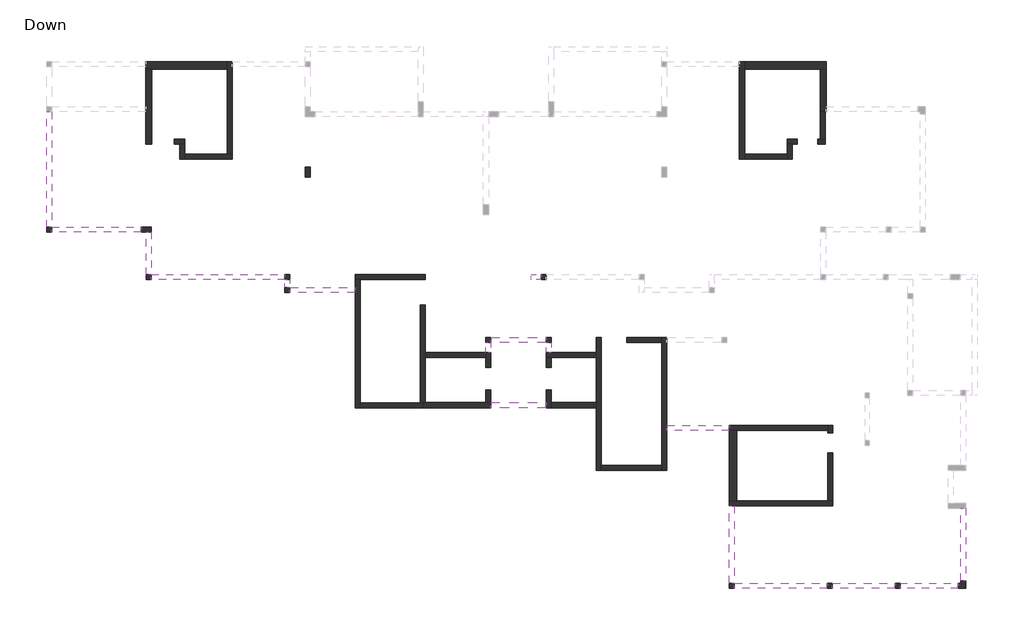
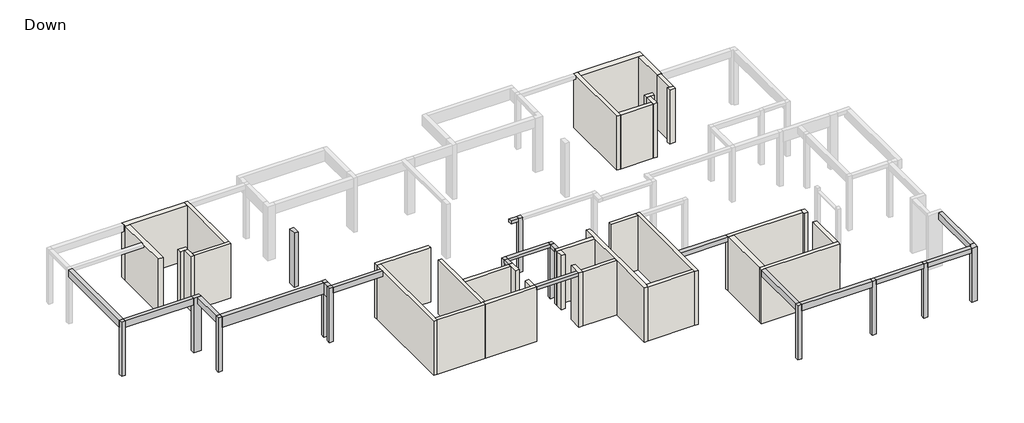
# One storey, part 1 of 2: 35 walls, 17 beams, 13 columns.
# Revit data of these elements (continued)
# Element 25 (IfcColumn, "Concrete Rectengular Column : 20/20") (continued)
#   SOFiSTiK_AMG_Adjusted = yes
#   Structural Material = Concrete
#   Phase Created = New Construction
#   Materials on its faces: "Concrete"
# Element 26 (IfcColumn, "Concrete Rectengular Column : 20/20")
#   Comments = ""
#   Mark = "C26"
#   SOFiSTiK_AMG_Comments = ""
#   SOFiSTiK_AMG_Scheduled = yes
#   SOFiSTiK_AMG_Adjusted = yes
#   Structural Material = Concrete
#   Phase Created = New Construction
#   Materials on its faces: "Concrete"
# Element 27 (IfcColumn, "Concrete Rectengular Column : 20/20")
#   Comments = ""
#   Mark = "C27"
#   SOFiSTiK_AMG_Comments = ""
#   SOFiSTiK_AMG_Scheduled = yes
#   SOFiSTiK_AMG_Adjusted = yes
#   Structural Material = Concrete
#   Phase Created = New Construction
#   Materials on its faces: "Concrete"
# Element 28 (IfcColumn, "Concrete Rectengular Column : 20/40")
#   Comments = ""
#   Mark = "C31"
#   SOFiSTiK_AMG_Comments = ""
#   SOFiSTiK_AMG_Scheduled = yes
#   SOFiSTiK_AMG_Adjusted = yes
#   Structural Material = Concrete
#   Phase Created = New Construction
#   Materials on its faces: "Concrete"
# Element 29 (IfcColumn, "Concrete Rectengular Column : 20/40")
#   Comments = ""
#   Mark = "C32"
#   SOFiSTiK_AMG_Comments = ""
#   SOFiSTiK_AMG_Scheduled = yes
#   SOFiSTiK_AMG_Adjusted = yes
#   Structural Material = Concrete
#   Phase Created = New Construction
#   Materials on its faces: "Concrete"
# Element 30 (IfcColumn, "L Column : 30/30/20/20")
#   Comments = ""
#   Mark = "C38"
#   SOFiSTiK_AMG_Comments = ""
#   SOFiSTiK_AMG_Scheduled = yes
#   SOFiSTiK_AMG_Adjusted = yes
#   Structural Material = Concrete
#   Phase Created = New Construction
# Element 31 (IfcWall, "20")
#   Comments = ""
#   Mark = "W1"
#   SOFiSTiK_AMG_Comments = ""
#   Top Offset = 0 cm
#   Base Offset = 0 cm
#   wall height = 300 cm
#   SOFiSTiK_AMG_Scheduled = yes
#   SOFiSTiK_AMG_Adjusted = yes
#   Phase Created = New Construction
#   Base Constraint = Down
#   Top Constraint = Typical Floor
#   Materials on its faces: "Concrete"
# Element 32 (IfcWall, "20")
#   Comments = ""
#   Mark = "W2"
#   SOFiSTiK_AMG_Comments = ""
#   Top Offset = 0 cm
#   Base Offset = 0 cm
#   wall height = 300 cm
#   SOFiSTiK_AMG_Scheduled = yes
#   SOFiSTiK_AMG_Adjusted = yes
#   Phase Created = New Construction
#   Base Constraint = Down
#   Top Constraint = Typical Floor
#   Materials on its faces: "Concrete"
# Element 33 (IfcWall, "20")
#   Comments = ""
#   Mark = "W3"
#   SOFiSTiK_AMG_Comments = ""
#   Top Offset = 0 cm
#   Base Offset = 0 cm
#   wall height = 300 cm
#   SOFiSTiK_AMG_Scheduled = yes
#   SOFiSTiK_AMG_Adjusted = yes
#   Phase Created = New Construction
#   Base Constraint = Down
#   Top Constraint = Typical Floor
#   Materials on its faces: "Concrete"
# Element 34 (IfcWall, "20")
#   Comments = ""
#   Mark = "W4"
#   SOFiSTiK_AMG_Comments = ""
#   Top Offset = 0 cm
#   Base Offset = 0 cm
#   wall height = 300 cm
#   SOFiSTiK_AMG_Scheduled = yes
#   SOFiSTiK_AMG_Adjusted = yes
#   Phase Created = New Construction
#   Base Constraint = Down
#   Top Constraint = Typical Floor
#   Materials on its faces: "Concrete"
# Element 35 (IfcWall, "20")
#   Comments = ""
#   Mark = "W5"
#   SOFiSTiK_AMG_Comments = ""
#   Top Offset = 0 cm
#   Base Offset = 0 cm
#   wall height = 300 cm
#   SOFiSTiK_AMG_Scheduled = yes
#   SOFiSTiK_AMG_Adjusted = yes
#   Phase Created = New Construction
#   Base Constraint = Down
#   Top Constraint = Typical Floor
#   Materials on its faces: "Concrete"
# Element 36 (IfcWall, "20")
#   Comments = ""
#   Mark = "W6"
#   SOFiSTiK_AMG_Comments = ""
#   Top Offset = 0 cm
#   Base Offset = 0 cm
#   wall height = 300 cm
#   SOFiSTiK_AMG_Scheduled = yes
#   SOFiSTiK_AMG_Adjusted = yes
#   Phase Created = New Construction
#   Base Constraint = Down
#   Top Constraint = Typical Floor
#   Materials on its faces: "Concrete"
# Element 37 (IfcWall, "20")
#   Comments = ""
#   Mark = "W7"
#   SOFiSTiK_AMG_Comments = ""
#   Top Offset = 0 cm
#   Base Offset = 0 cm
#   wall height = 300 cm
#   SOFiSTiK_AMG_Scheduled = yes
#   SOFiSTiK_AMG_Adjusted = yes
#   Phase Created = New Construction
#   Base Constraint = Down
#   Top Constraint = Typical Floor
#   Materials on its faces: "Concrete"
# Element 38 (IfcWall, "20")
#   Comments = ""
#   Mark = "W8"
#   SOFiSTiK_AMG_Comments = ""
#   Top Offset = 0 cm
#   Base Offset = 0 cm
#   wall height = 300 cm
#   SOFiSTiK_AMG_Scheduled = yes
#   SOFiSTiK_AMG_Adjusted = yes
#   Phase Created = New Construction
#   Base Constraint = Down
#   Top Constraint = Typical Floor
#   Materials on its faces: "Concrete"
# Element 39 (IfcWall, "20")
#   Comments = ""
#   Mark = "W9"
#   SOFiSTiK_AMG_Comments = ""
#   Top Offset = 0 cm
#   Base Offset = 0 cm
#   wall height = 300 cm
#   SOFiSTiK_AMG_Scheduled = yes
#   SOFiSTiK_AMG_Adjusted = yes
#   Phase Created = New Construction
#   Base Constraint = Down
#   Top Constraint = Typical Floor
#   Materials on its faces: "Concrete"
# Element 40 (IfcWall, "20")
#   Comments = ""
#   Mark = "W10"
#   SOFiSTiK_AMG_Comments = ""
#   Top Offset = 0 cm
#   Base Offset = 0 cm
#   wall height = 300 cm
#   SOFiSTiK_AMG_Scheduled = yes
#   SOFiSTiK_AMG_Adjusted = yes
#   Phase Created = New Construction
#   Base Constraint = Down
#   Top Constraint = Typical Floor
#   Materials on its faces: "Concrete"
# Element 41 (IfcWall, "20")
#   Comments = ""
#   Mark = "W11"
#   SOFiSTiK_AMG_Comments = ""
#   Top Offset = 0 cm
#   Base Offset = 0 cm
#   wall height = 300 cm
#   SOFiSTiK_AMG_Scheduled = yes
#   SOFiSTiK_AMG_Adjusted = yes
#   Phase Created = New Construction
#   Base Constraint = Down
#   Top Constraint = Typical Floor
#   Materials on its faces: "Concrete"
# Element 42 (IfcWall, "20")
#   Comments = ""
#   Mark = "W12"
#   SOFiSTiK_AMG_Comments = ""
#   Top Offset = 0 cm
#   Base Offset = 0 cm
#   wall height = 300 cm
#   SOFiSTiK_AMG_Scheduled = yes
#   SOFiSTiK_AMG_Adjusted = yes
#   Phase Created = New Construction
#   Base Constraint = Down
#   Top Constraint = Typical Floor
#   Materials on its faces: "Concrete"
# Element 43 (IfcWall, "20")
#   Comments = ""
#   Mark = "W13"
#   SOFiSTiK_AMG_Comments = ""
#   Top Offset = 0 cm
#   Base Offset = 0 cm
#   wall height = 300 cm
#   SOFiSTiK_AMG_Scheduled = yes
#   SOFiSTiK_AMG_Adjusted = yes
#   Phase Created = New Construction
#   Base Constraint = Down
#   Top Constraint = Typical Floor
#   Materials on its faces: "Concrete"
# Element 44 (IfcWall, "20")
#   Comments = ""
#   Mark = "W14"
#   SOFiSTiK_AMG_Comments = ""
#   Top Offset = 0 cm
#   Base Offset = 0 cm
#   wall height = 300 cm
#   SOFiSTiK_AMG_Scheduled = yes
#   SOFiSTiK_AMG_Adjusted = yes
#   Phase Created = New Construction
#   Base Constraint = Down
#   Top Constraint = Typical Floor
#   Materials on its faces: "Concrete"
# Element 45 (IfcWall, "20")
#   Comments = ""
#   Mark = "W15"
#   SOFiSTiK_AMG_Comments = ""
#   Top Offset = 0 cm
#   Base Offset = 0 cm
#   wall height = 300 cm
#   SOFiSTiK_AMG_Scheduled = yes
#   SOFiSTiK_AMG_Adjusted = yes
#   Phase Created = New Construction
#   Base Constraint = Down
#   Top Constraint = Typical Floor
#   Materials on its faces: "Concrete"
# Element 46 (IfcWall, "20")
#   Comments = ""
#   Mark = "W16"
#   SOFiSTiK_AMG_Comments = ""
#   Top Offset = 0 cm
#   Base Offset = 0 cm
#   wall height = 300 cm
#   SOFiSTiK_AMG_Scheduled = yes
#   SOFiSTiK_AMG_Adjusted = yes
#   Phase Created = New Construction
#   Base Constraint = Down
#   Top Constraint = Typical Floor
#   Materials on its faces: "Concrete"
# Element 47 (IfcWall, "20")
#   Comments = ""
#   Mark = "W17"
#   SOFiSTiK_AMG_Comments = ""
#   Top Offset = 0 cm
#   Base Offset = 0 cm
#   wall height = 300 cm
#   SOFiSTiK_AMG_Scheduled = yes
#   SOFiSTiK_AMG_Adjusted = yes
#   Phase Created = New Construction
#   Base Constraint = Down
#   Top Constraint = Typical Floor
#   Materials on its faces: "Concrete"
# Element 48 (IfcWall, "20")
#   Comments = ""
#   Mark = "W18"
#   SOFiSTiK_AMG_Comments = ""
#   Top Offset = 0 cm
#   Base Offset = 0 cm
#   wall height = 300 cm
#   SOFiSTiK_AMG_Scheduled = yes
#   SOFiSTiK_AMG_Adjusted = yes
#   Phase Created = New Construction
#   Base Constraint = Down
#   Top Constraint = Typical Floor
#   Materials on its faces: "Concrete"
# Element 49 (IfcWall, "20")
#   Comments = ""
#   Mark = "W19"
#   SOFiSTiK_AMG_Comments = ""
#   Top Offset = 0 cm
#   Base Offset = 0 cm
#   wall height = 300 cm
#   SOFiSTiK_AMG_Scheduled = yes
#   SOFiSTiK_AMG_Adjusted = yes
#   Phase Created = New Construction
#   Base Constraint = Down
#   Top Constraint = Typical Floor
#   Materials on its faces: "Concrete"
# Element 50 (IfcWall, "20")
#   Comments = ""
#   Mark = "W20"
#   SOFiSTiK_AMG_Comments = ""
#   Top Offset = 0 cm
#   Base Offset = 0 cm
#   wall height = 300 cm
#   SOFiSTiK_AMG_Scheduled = yes
#   SOFiSTiK_AMG_Adjusted = yes
#   Phase Created = New Construction
#   Base Constraint = Down
#   Top Constraint = Typical Floor
#   Materials on its faces: "Concrete"
# Element 51 (IfcWall, "20")
#   Comments = ""
#   Mark = "W21"
#   SOFiSTiK_AMG_Comments = ""
#   Top Offset = 0 cm
#   Base Offset = 0 cm
#   wall height = 300 cm
#   SOFiSTiK_AMG_Scheduled = yes
#   SOFiSTiK_AMG_Adjusted = yes
#   Phase Created = New Construction
#   Base Constraint = Down
#   Top Constraint = Typical Floor
#   Materials on its faces: "Concrete"
# Element 52 (IfcWall, "20")
#   Comments = ""
#   Mark = "W22"
#   SOFiSTiK_AMG_Comments = ""
#   Top Offset = 0 cm
#   Base Offset = 0 cm
#   wall height = 300 cm
#   SOFiSTiK_AMG_Scheduled = yes
#   SOFiSTiK_AMG_Adjusted = yes
#   Phase Created = New Construction
#   Base Constraint = Down
#   Top Constraint = Typical Floor
#   Materials on its faces: "Concrete"
# Element 53 (IfcWall, "20")
#   Comments = ""
#   Mark = "W23"
#   SOFiSTiK_AMG_Comments = ""
#   Top Offset = 0 cm
#   Base Offset = 0 cm
#   wall height = 300 cm
#   SOFiSTiK_AMG_Scheduled = yes
#   SOFiSTiK_AMG_Adjusted = yes
#   Phase Created = New Construction
#   Base Constraint = Down
#   Top Constraint = Typical Floor
#   Materials on its faces: "Concrete"
# Element 54 (IfcWall, "20")
#   Comments = ""
#   Mark = "W24"
#   SOFiSTiK_AMG_Comments = ""
#   Top Offset = 0 cm
#   Base Offset = 0 cm
#   wall height = 300 cm
#   SOFiSTiK_AMG_Scheduled = yes
#   SOFiSTiK_AMG_Adjusted = yes
#   Phase Created = New Construction
#   Base Constraint = Down
#   Top Constraint = Typical Floor
#   Materials on its faces: "Concrete"
# Element 55 (IfcWall, "20")
#   Comments = ""
#   Mark = "W25"
#   SOFiSTiK_AMG_Comments = ""
#   Top Offset = 0 cm
#   Base Offset = 0 cm
#   wall height = 300 cm
#   SOFiSTiK_AMG_Scheduled = yes
#   SOFiSTiK_AMG_Adjusted = yes
#   Phase Created = New Construction
#   Base Constraint = Down
#   Top Constraint = Typical Floor
#   Materials on its faces: "Concrete"
# Element 56 (IfcWall, "20")
#   Comments = ""
#   Mark = "W26"
#   SOFiSTiK_AMG_Comments = ""
#   Top Offset = 0 cm
#   Base Offset = 0 cm
#   wall height = 300 cm
#   SOFiSTiK_AMG_Scheduled = yes
#   SOFiSTiK_AMG_Adjusted = yes
#   Phase Created = New Construction
#   Base Constraint = Down
#   Top Constraint = Typical Floor
#   Materials on its faces: "Concrete"
# Element 57 (IfcWall, "20")
#   Comments = ""
#   Mark = "W27"
#   SOFiSTiK_AMG_Comments = ""
#   Top Offset = 0 cm
#   Base Offset = 0 cm
#   wall height = 300 cm
#   SOFiSTiK_AMG_Scheduled = yes
#   SOFiSTiK_AMG_Adjusted = yes
#   Phase Created = New Construction
#   Base Constraint = Down
#   Top Constraint = Typical Floor
#   Materials on its faces: "Concrete"
# Element 58 (IfcWall, "20")
#   Comments = ""
#   Mark = "W28"
#   SOFiSTiK_AMG_Comments = ""
#   Top Offset = 0 cm
#   Base Offset = 0 cm
#   wall height = 300 cm
#   SOFiSTiK_AMG_Scheduled = yes
#   SOFiSTiK_AMG_Adjusted = yes
#   Phase Created = New Construction
#   Base Constraint = Down
#   Top Constraint = Typical Floor
#   Materials on its faces: "Concrete"
# Element 59 (IfcWall, "20")
#   Comments = ""
#   Mark = "W29"
#   SOFiSTiK_AMG_Comments = ""
#   Top Offset = 0 cm
#   Base Offset = 0 cm
#   wall height = 300 cm
#   SOFiSTiK_AMG_Scheduled = yes
#   SOFiSTiK_AMG_Adjusted = yes
#   Phase Created = New Construction
#   Base Constraint = Down
#   Top Constraint = Typical Floor
#   Materials on its faces: "Concrete"
# Element 60 (IfcWall, "20")
#   Comments = ""
#   Mark = "W30"
#   SOFiSTiK_AMG_Comments = ""
#   Top Offset = 0 cm
#   Base Offset = 0 cm
#   wall height = 300 cm
#   SOFiSTiK_AMG_Scheduled = yes
#   SOFiSTiK_AMG_Adjusted = yes
#   Phase Created = New Construction
#   Base Constraint = Down
#   Top Constraint = Typical Floor
#   Materials on its faces: "Concrete"
# Element 61 (IfcWall, "25")
#   Comments = ""
#   Mark = "W34"
#   SOFiSTiK_AMG_Comments = ""
#   Top Offset = 0 cm
#   Base Offset = 0 cm
#   wall height = 300 cm
#   SOFiSTiK_AMG_Scheduled = yes
#   SOFiSTiK_AMG_Adjusted = yes
#   Phase Created = New Construction
#   Base Constraint = Down
#   Top Constraint = Typical Floor
#   Materials on its faces: "Concrete"
# Element 62 (IfcWall, "25")
#   Comments = ""
#   Mark = "W35"
#   SOFiSTiK_AMG_Comments = ""
#   Top Offset = 0 cm
#   Base Offset = 0 cm
#   wall height = 300 cm
#   SOFiSTiK_AMG_Scheduled = yes
#   SOFiSTiK_AMG_Adjusted = yes
#   Phase Created = New Construction
#   Base Constraint = Down
#   Top Constraint = Typical Floor
#   Materials on its faces: "Concrete"
# Element 63 (IfcWall, "30")
#   Comments = ""
#   Mark = "W31"
#   SOFiSTiK_AMG_Comments = ""
#   Top Offset = 0 cm
#   Base Offset = 0 cm
#   wall height = 300 cm
#   SOFiSTiK_AMG_Scheduled = yes
#   SOFiSTiK_AMG_Adjusted = yes
#   Phase Created = New Construction
#   Base Constraint = Down
#   Top Constraint = Typical Floor
#   Materials on its faces: "Concrete"
# Element 64 (IfcWall, "30")
#   Comments = ""
#   Mark = "W32"
#   SOFiSTiK_AMG_Comments = ""
#   Top Offset = 0 cm
#   Base Offset = 0 cm
#   wall height = 300 cm
#   SOFiSTiK_AMG_Scheduled = yes
#   SOFiSTiK_AMG_Adjusted = yes
#   Phase Created = New Construction
#   Base Constraint = Down
#   Top Constraint = Typical Floor
#   Materials on its faces: "Concrete"
# Element 65 (IfcWall, "30")
#   Comments = ""
#   Mark = "W33"
#   SOFiSTiK_AMG_Comments = ""
#   Top Offset = 0 cm
#   Base Offset = 0 cm
#   wall height = 300 cm
#   SOFiSTiK_AMG_Scheduled = yes
#   SOFiSTiK_AMG_Adjusted = yes
#   Phase Created = New Construction
#   Base Constraint = Down
#   Top Constraint = Typical Floor
#   Materials on its faces: "Concrete"
# Materials
#   "Concrete": class "Concrete", colour RGB 192 192 192, transparency 0, Keynote = "01000", Description = "Cast-in-place concrete", Cost = 0
#   "Concrete, Cast-in-Place gray": class "Concrete", colour RGB 192 192 192, transparency 0, Description = "Cast-in-place concrete", Cost = 0
